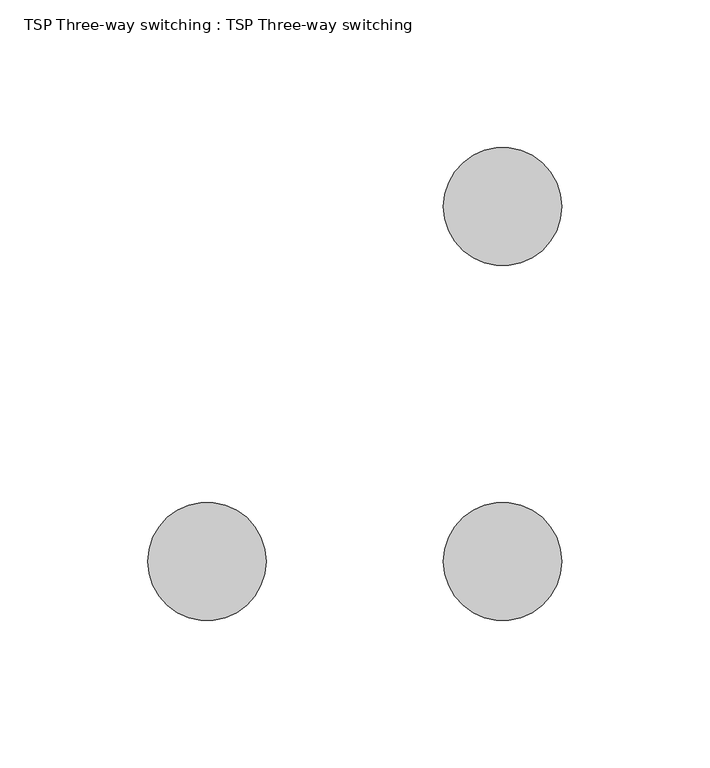
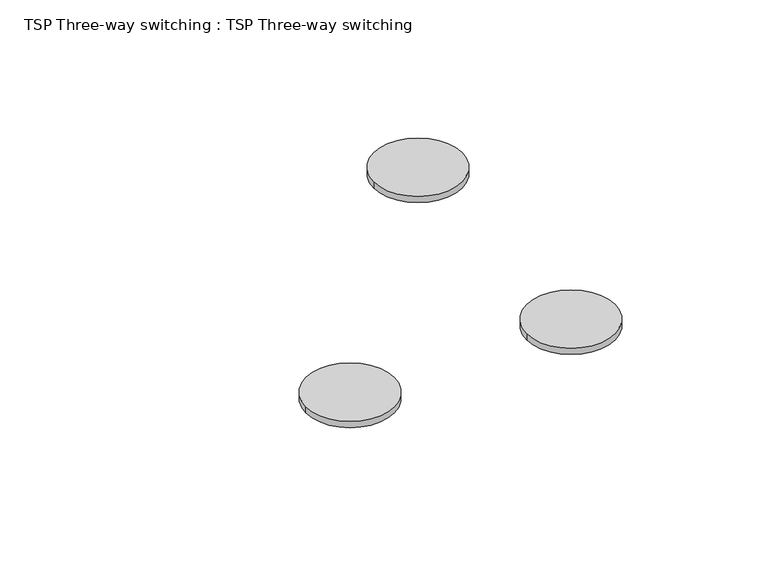
"""IFC4 building model written with IfcOpenShell, lengths in millimetres: proxy geometry, TSP Three-way switching : TSP Three-way switching."""

from ifc_helpers import new_model, si_unit, point, frame_2d, origin, origin_with_axes, place, context, project, spatial, circle_curve, trimmed, segment, composite_curve, outline, extrude, source, transform, mapped, element, save


def tsp_three_way_switching_tsp_three_way_switching_a70eb910(model_context):
    return source(origin(), model_context, "Body", "SweptSolid", [
        extrude(outline(composite_curve([segment(trimmed(circle_curve(frame_2d((50.0, 60.0)), 20.0), [point((70.0, 60.0))], [point((30.0, 60.0))], False, "CARTESIAN"), True, "CONTINUOUS"), segment(trimmed(circle_curve(frame_2d((50.0, 60.0)), 20.0), [point((30.0, 60.0))], [point((70.0, 60.0))], False, "CARTESIAN"), True, "CONTINUOUS")], self_intersect=False)), origin_with_axes(), (0.0, 0.0, 1.0), 3.0),
        extrude(outline(composite_curve([segment(trimmed(circle_curve(frame_2d((-50.0, -60.0)), 20.0), [point((-70.0, -60.0))], [point((-30.0, -60.0))], False, "CARTESIAN"), True, "CONTINUOUS"), segment(trimmed(circle_curve(frame_2d((-50.0, -60.0)), 20.0), [point((-30.0, -60.0))], [point((-70.0, -60.0))], False, "CARTESIAN"), True, "CONTINUOUS")], self_intersect=False)), origin_with_axes(), (0.0, 0.0, 1.0), 3.0),
        extrude(outline(composite_curve([segment(trimmed(circle_curve(frame_2d((50.0, -60.0)), 20.0), [point((70.0, -60.0))], [point((30.0, -60.0))], False, "CARTESIAN"), True, "CONTINUOUS"), segment(trimmed(circle_curve(frame_2d((50.0, -60.0)), 20.0), [point((30.0, -60.0))], [point((70.0, -60.0))], False, "CARTESIAN"), True, "CONTINUOUS")], self_intersect=False)), origin_with_axes(), (0.0, 0.0, 1.0), 3.0),
    ])


if __name__ == "__main__":
    model = new_model("IFC4")
    model_context = context("Model", 3, world=origin())
    ifc_project = project(units=[si_unit("LENGTHUNIT", "METRE", prefix="MILLI")], contexts=[model_context])
    site = spatial("IfcSite", under=ifc_project)
    building = spatial("IfcBuilding", under=site)
    placement = place(None, origin())
    tsp_three_way_switching_tsp_three_way_switching_shape = tsp_three_way_switching_tsp_three_way_switching_a70eb910(model_context)
    element("IfcBuildingElementProxy", 1, Name="TSP Three-way switching : TSP Three-way switching", ObjectType="TSP Three-way switching : TSP Three-way switching", at=placement, inside=building, context=model_context, shape_type="MappedRepresentation", body=[
        mapped(tsp_three_way_switching_tsp_three_way_switching_shape, transform((0.0, 0.0, 0.0), x_axis=(1.0, 0.0, 0.0), y_axis=(0.0, 1.0, 0.0), z_axis=(0.0, 0.0, 1.0))),
    ])
    save(model, "model.ifc")

# Revit data of these elements
# Type "TSP Three-way switching : TSP Three-way switching"
#   Model = "TSP_ELEC3WS"
#   Default Elevation = 0
# Element 1 (IfcBuildingElementProxy, "TSP Three-way switching : TSP Three-way switching")
#   Materials on its faces: "Plastic, Opaque Black"
# Materials
#   "Plastic, Opaque Black": class "Plastic", colour RGB 0 0 0, transparency 0.7, Description = "Plastic, generic, opaque black", Cost = 0
